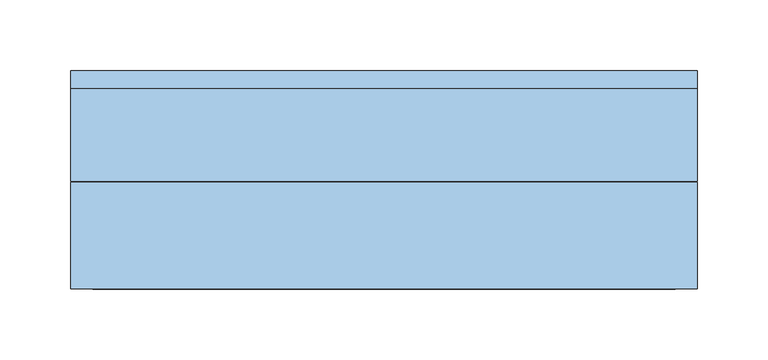
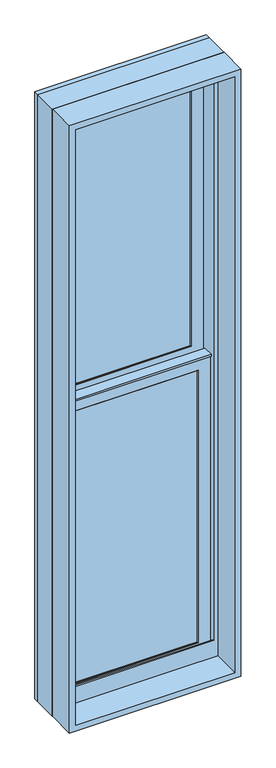
"""IFC4 building model written with IfcOpenShell, lengths in millimetres: window geometry, Window-Double_Hung-Marvin-Essential : ESDH1656."""

from ifc_helpers import new_model, si_unit, frame, origin, place, context, project, spatial, polyline, outline, extrude, faceted_brep, source, transform, mapped, element, save


def window_900ccffd(model_context):
    return source(origin(), model_context, "Body", "SolidModel", [
        extrude(outline(polyline([(64.5583333, 20.6375), (64.5583333, 15.875), (45.5083333, 15.875), (45.5083333, 20.6375), (64.5583333, 20.6375)])), frame((0.0, 0.0, 831.85), z_axis=(0.0, 0.0, 1.0), x_axis=(1.0, 0.0, 0.0)), (0.0, 0.0, 1.0), 755.65),
        extrude(outline(polyline([(-45.5083333, 20.6375), (-45.5083333, 15.875), (-64.5583333, 15.875), (-64.5583333, 20.6375), (-45.5083333, 20.6375)])), frame((0.0, 0.0, 831.85), z_axis=(0.0, 0.0, 1.0), x_axis=(1.0, 0.0, 0.0)), (0.0, 0.0, 1.0), 755.65),
        extrude(outline(polyline([(165.1, 20.6375), (165.1, 15.875), (-165.1, 15.875), (-165.1, 20.6375), (165.1, 20.6375)])), frame((0.0, 0.0, 1200.15), z_axis=(0.0, 0.0, 1.0), x_axis=(1.0, 0.0, 0.0)), (0.0, 0.0, 1.0), 19.05),
        extrude(outline(polyline([(-64.5583333, 46.83125), (-64.5583333, 51.59375), (-45.5083333, 51.59375), (-45.5083333, 46.83125), (-64.5583333, 46.83125)])), frame((0.0, 0.0, 1625.6), z_axis=(0.0, 0.0, 1.0), x_axis=(1.0, 0.0, 0.0)), (0.0, 0.0, 1.0), 755.65),
        extrude(outline(polyline([(45.5083333, 46.83125), (45.5083333, 51.59375), (64.5583333, 51.59375), (64.5583333, 46.83125), (45.5083333, 46.83125)])), frame((0.0, 0.0, 1625.6), z_axis=(0.0, 0.0, 1.0), x_axis=(1.0, 0.0, 0.0)), (0.0, 0.0, 1.0), 755.65),
        extrude(outline(polyline([(-165.1, 46.83125), (-165.1, 51.59375), (165.1, 51.59375), (165.1, 46.83125), (-165.1, 46.83125)])), frame((0.0, 0.0, 1993.9), z_axis=(0.0, 0.0, 1.0), x_axis=(1.0, 0.0, 0.0)), (0.0, 0.0, 1.0), 19.05),
        extrude(outline(polyline([(64.5583333, 20.6375), (45.5083333, 20.6375), (45.5083333, 25.4), (64.5583333, 25.4), (64.5583333, 20.6375)])), frame((0.0, 0.0, 831.85), z_axis=(0.0, 0.0, 1.0), x_axis=(1.0, 0.0, 0.0)), (0.0, 0.0, 1.0), 755.65),
        extrude(outline(polyline([(-45.5083333, 20.6375), (-64.5583333, 20.6375), (-64.5583333, 25.4), (-45.5083333, 25.4), (-45.5083333, 20.6375)])), frame((0.0, 0.0, 831.85), z_axis=(0.0, 0.0, 1.0), x_axis=(1.0, 0.0, 0.0)), (0.0, 0.0, 1.0), 755.65),
        extrude(outline(polyline([(165.1, 20.6375), (-165.1, 20.6375), (-165.1, 25.4), (165.1, 25.4), (165.1, 20.6375)])), frame((0.0, 0.0, 1200.15), z_axis=(0.0, 0.0, 1.0), x_axis=(1.0, 0.0, 0.0)), (0.0, 0.0, 1.0), 19.05),
        extrude(outline(polyline([(-64.5583333, 56.35625), (-45.5083333, 56.35625), (-45.5083333, 51.59375), (-64.5583333, 51.59375), (-64.5583333, 56.35625)])), frame((0.0, 0.0, 1625.6), z_axis=(0.0, 0.0, 1.0), x_axis=(1.0, 0.0, 0.0)), (0.0, 0.0, 1.0), 755.65),
        extrude(outline(polyline([(45.5083333, 56.35625), (64.5583333, 56.35625), (64.5583333, 51.59375), (45.5083333, 51.59375), (45.5083333, 56.35625)])), frame((0.0, 0.0, 1625.6), z_axis=(0.0, 0.0, 1.0), x_axis=(1.0, 0.0, 0.0)), (0.0, 0.0, 1.0), 755.65),
        extrude(outline(polyline([(-165.1, 56.35625), (165.1, 56.35625), (165.1, 51.59375), (-165.1, 51.59375), (-165.1, 56.35625)])), frame((0.0, 0.0, 1993.9), z_axis=(0.0, 0.0, 1.0), x_axis=(1.0, 0.0, 0.0)), (0.0, 0.0, 1.0), 19.05),
        faceted_brep([(-192.0875, 5.6780605, 1617.5351748), (-192.0875, 5.6780605, 1612.9), (192.0875, 5.6780605, 1612.9), (192.0875, 5.6780605, 1617.5351748), (-192.0875, 34.8118605, 1617.5351748), (192.0875, 34.8118605, 1617.5351748), (192.0875, 34.8118605, 1612.9), (-192.0875, 34.8118605, 1612.9), (-192.0875, 30.1625, 1612.9), (-192.0875, 30.1625, 804.8625), (-192.0875, 8.9241104, 804.8625), (-192.0875, 8.9241104, 1612.9), (192.0875, 8.9241104, 1612.9), (192.0875, 30.1625, 1612.9), (192.0875, 8.9241104, 804.8625), (192.0875, 30.1625, 804.8625), (-176.2034752, 11.90625, 1598.6034752), (-176.2034752, 30.1625, 1598.6034752), (176.2034752, 30.1625, 1598.6034752), (176.2034752, 11.90625, 1598.6034752), (-159.54375, 10.4662439, 1581.94375), (-159.54375, 11.90625, 1581.94375), (159.54375, 11.90625, 1581.94375), (159.54375, 10.4662439, 1581.94375), (161.0858834, 8.9241104, 1583.4858834), (-161.0858834, 8.9241104, 1583.4858834), (176.2034752, 30.1625, 820.7465248), (176.2034752, 11.90625, 820.7465248), (159.54375, 11.90625, 837.40625), (159.54375, 10.4662439, 837.40625), (161.0858834, 8.9241104, 835.8641166), (-176.2034752, 30.1625, 820.7465248), (-176.2034752, 11.90625, 820.7465248), (-159.54375, 11.90625, 837.40625), (-159.54375, 10.4662439, 837.40625), (-161.0858834, 8.9241104, 835.8641166)], [[[0, 1, 2, 3]], [[4, 5, 6, 7]], [[1, 0, 4, 7, 8, 9, 10, 11]], [[2, 1, 11, 12]], [[7, 6, 13, 8]], [[3, 2, 12, 14, 15, 13, 6, 5]], [[0, 3, 5, 4]], [[16, 17, 18, 19]], [[20, 21, 22, 23]], [[20, 23, 24, 25]], [[19, 18, 26, 27]], [[23, 22, 28, 29]], [[24, 23, 29, 30]], [[27, 26, 31, 32]], [[29, 28, 33, 34]], [[30, 29, 34, 35]], [[15, 14, 10, 9]], [[15, 9, 8, 13], [18, 17, 31, 26]], [[17, 16, 32, 31]], [[16, 19, 27, 32], [22, 21, 33, 28]], [[21, 20, 34, 33]], [[20, 25, 35, 34]], [[10, 14, 12, 11], [25, 24, 30, 35]]]),
        extrude(outline(polyline([(38.5955581, 1598.6125), (33.5778968, 1598.6125), (33.5778968, 1600.2), (39.9405976, 1600.2), (39.9405976, 1598.6125), (61.515625, 1598.6125), (47.6307501, 1595.2975159), (38.5955581, 1595.2975159), (38.5955581, 1598.6125)])), frame((-192.0875, 0.0, 0.0), z_axis=(1.0, 0.0, 0.0), x_axis=(0.0, 1.0, 0.0)), (0.0, 0.0, 1.0), 384.175),
        faceted_brep([(222.25, 0.0, 774.7), (222.25, 0.0, 2438.4), (-222.25, 0.0, 2438.4), (-222.25, 0.0, 774.7), (196.05625, 0.0, 835.81875), (-196.05625, 0.0, 835.81875), (-196.05625, 0.0, 2412.20625), (196.05625, 0.0, 2412.20625), (196.05625, 3.96875, 774.7), (-196.05625, 3.96875, 774.7), (-196.05625, 3.96875, 835.81875), (196.05625, 3.96875, 835.81875), (-222.25, 65.6828125, 774.7), (-196.05625, 65.6828125, 774.7), (196.05625, 65.6828125, 774.7), (222.25, 65.6828125, 774.7), (-222.25, 65.6828125, 2438.4), (222.25, 65.6828125, 2438.4), (196.05625, 65.6828125, 2412.20625), (-196.05625, 65.6828125, 2412.20625)], [[[0, 1, 2, 3], [4, 5, 6, 7]], [[8, 9, 10, 11]], [[5, 4, 11, 10]], [[0, 3, 12, 13, 9, 8, 14, 15]], [[13, 12, 16, 17, 15, 14, 18, 19]], [[13, 19, 6, 5, 10, 9]], [[7, 6, 19, 18]], [[18, 14, 8, 11, 4, 7]], [[1, 0, 15, 17]], [[2, 1, 17, 16]], [[3, 2, 16, 12]]]),
        faceted_brep([(196.05625, 30.1625, 1606.55), (194.46875, 30.1625, 1606.55), (194.46875, 30.1625, 799.0544613), (196.05625, 30.1625, 799.0544613), (-194.46875, 30.1625, 1606.55), (-196.05625, 30.1625, 1606.55), (-196.05625, 30.1625, 799.0544613), (-194.46875, 30.1625, 799.0544613), (194.46875, 63.5, 1606.55), (196.05625, 63.5, 1606.55), (196.05625, 63.5, 792.5743077), (194.46875, 63.5, 792.5743077), (-196.05625, 63.5, 1606.55), (-194.46875, 63.5, 1606.55), (-194.46875, 63.5, 792.5743077), (-196.05625, 63.5, 792.5743077), (207.3108932, 3.96875, 804.1460105), (207.3108932, 3.96875, 774.7), (207.3108932, 65.6828125, 774.7), (207.3108932, 65.6828125, 792.150012), (-207.3108932, 3.96875, 774.7), (-207.3108932, 3.96875, 804.1460105), (-207.3108932, 65.6828125, 792.150012), (-207.3108932, 65.6828125, 774.7), (207.3108932, 78.58125, 789.6428097), (-207.3108932, 78.58125, 789.6428097), (-205.2971252, 68.2348864, 791.6539391), (-187.33135, 68.2348864, 791.6539391), (-187.33135, 65.6828125, 792.150012), (187.33135, 65.6828125, 792.150012), (187.33135, 68.2348864, 791.6539391), (205.2971252, 68.2348864, 791.6539391), (-222.25, 65.6828125, 774.7), (-222.25, 78.5948249, 774.7), (222.25, 78.5948249, 774.7), (222.25, 65.6828125, 774.7), (-222.25, 78.58125, 2438.4), (222.25, 78.58125, 2438.4), (207.3108932, 78.58125, 2423.4608932), (-207.3108932, 78.58125, 2423.4608932), (-222.25, 65.6828125, 2438.4), (-205.2971252, 68.2348864, 2421.4471252), (205.2971252, 68.2348864, 2421.4471252), (187.33135, 68.2348864, 2403.48135), (-187.33135, 68.2348864, 2403.48135), (-187.33135, 65.6828125, 2403.48135), (187.33135, 65.6828125, 2403.48135), (222.25, 65.6828125, 2438.4)], [[[0, 1, 2, 3]], [[4, 5, 6, 7]], [[8, 9, 10, 11]], [[12, 13, 14, 15]], [[1, 8, 11, 2]], [[9, 0, 3, 10]], [[1, 0, 9, 8]], [[5, 4, 13, 12]], [[5, 12, 15, 6]], [[13, 4, 7, 14]], [[16, 17, 18, 19]], [[20, 21, 22, 23]], [[24, 25, 26, 27, 28, 22, 21, 16, 19, 29, 30, 31], [3, 2, 11, 10], [7, 6, 15, 14]], [[17, 16, 21, 20]], [[17, 20, 23, 32, 33, 34, 35, 18]], [[34, 33, 36, 37], [25, 24, 38, 39]], [[33, 32, 40, 36]], [[39, 41, 26, 25]], [[41, 42, 31, 30, 43, 44, 27, 26]], [[44, 45, 28, 27]], [[40, 32, 23, 22, 28, 45, 46, 29, 19, 18, 35, 47]], [[36, 40, 47, 37]], [[39, 38, 42, 41]], [[44, 43, 46, 45]], [[34, 37, 47, 35]], [[42, 38, 24, 31]], [[46, 43, 30, 29]]]),
        extrude(outline(polyline([(172.24375, 11.90625), (-172.24375, 11.90625), (-172.24375, 15.08125), (172.24375, 15.08125), (172.24375, 11.90625)])), frame((0.0, 0.0, 824.70625), z_axis=(0.0, 0.0, 1.0), x_axis=(1.0, 0.0, 0.0)), (0.0, 0.0, 1.0), 769.9375),
        extrude(outline(polyline([(172.24375, 42.8625), (-172.24375, 42.8625), (-172.24375, 46.0375), (172.24375, 46.0375), (172.24375, 42.8625)])), frame((0.0, 0.0, 1618.45625), z_axis=(0.0, 0.0, 1.0), x_axis=(1.0, 0.0, 0.0)), (0.0, 0.0, 1.0), 769.9375),
        faceted_brep([(-159.54375, 31.194477, 1581.94375), (-161.0858834, 32.7366104, 1583.4858834), (161.0858834, 32.7366104, 1583.4858834), (159.54375, 31.194477, 1581.94375), (-159.54375, 30.1625, 1581.94375), (159.54375, 30.1625, 1581.94375), (-192.0875, 32.7366104, 1614.4875), (-192.0875, 30.1625, 1614.4875), (192.0875, 30.1625, 1614.4875), (192.0875, 32.7366104, 1614.4875), (161.0858834, 32.7366104, 835.8641166), (159.54375, 31.194477, 837.40625), (159.54375, 30.1625, 837.40625), (192.0875, 30.1625, 804.8625), (192.0875, 32.7366104, 804.8625), (-161.0858834, 32.7366104, 835.8641166), (-159.54375, 31.194477, 837.40625), (-159.54375, 30.1625, 837.40625), (-192.0875, 30.1625, 804.8625), (-192.0875, 32.7366104, 804.8625)], [[[0, 1, 2, 3]], [[4, 0, 3, 5]], [[6, 7, 8, 9]], [[3, 2, 10, 11]], [[5, 3, 11, 12]], [[9, 8, 13, 14]], [[11, 10, 15, 16]], [[12, 11, 16, 17]], [[14, 13, 18, 19]], [[9, 14, 19, 6], [1, 15, 10, 2]], [[16, 15, 1, 0]], [[17, 16, 0, 4]], [[7, 18, 13, 8], [5, 12, 17, 4]], [[19, 18, 7, 6]]]),
        faceted_brep([(-176.2034752, 42.8625, 2392.3534752), (-176.2034752, 61.11875, 2392.3534752), (176.2034752, 61.11875, 2392.3534752), (176.2034752, 42.8625, 2392.3534752), (-159.54375, 41.4224939, 2375.69375), (-159.54375, 42.8625, 2375.69375), (159.54375, 42.8625, 2375.69375), (159.54375, 41.4224939, 2375.69375), (-161.0858834, 39.8803604, 2377.2358834), (161.0858834, 39.8803604, 2377.2358834), (-192.0875, 61.11875, 2408.2375), (-192.0875, 39.8803604, 2408.2375), (192.0875, 39.8803604, 2408.2375), (192.0875, 61.11875, 2408.2375), (176.2034752, 61.11875, 1614.4965248), (176.2034752, 42.8625, 1614.4965248), (159.54375, 42.8625, 1631.15625), (159.54375, 41.4224939, 1631.15625), (161.0858834, 39.8803604, 1629.6141166), (192.0875, 39.8803604, 1598.6125), (192.0875, 61.11875, 1598.6125), (-176.2034752, 61.11875, 1614.4965248), (-176.2034752, 42.8625, 1614.4965248), (-159.54375, 42.8625, 1631.15625), (-159.54375, 41.4224939, 1631.15625), (-161.0858834, 39.8803604, 1629.6141166), (-192.0875, 39.8803604, 1598.6125), (-192.0875, 61.11875, 1598.6125)], [[[0, 1, 2, 3]], [[4, 5, 6, 7]], [[8, 4, 7, 9]], [[10, 11, 12, 13]], [[3, 2, 14, 15]], [[7, 6, 16, 17]], [[9, 7, 17, 18]], [[13, 12, 19, 20]], [[15, 14, 21, 22]], [[17, 16, 23, 24]], [[18, 17, 24, 25]], [[20, 19, 26, 27]], [[13, 20, 27, 10], [1, 21, 14, 2]], [[22, 21, 1, 0]], [[3, 15, 22, 0], [5, 23, 16, 6]], [[24, 23, 5, 4]], [[25, 24, 4, 8]], [[11, 26, 19, 12], [9, 18, 25, 8]], [[27, 26, 11, 10]]]),
        faceted_brep([(-192.0875, 61.11875, 1598.6125), (-192.0875, 63.6928604, 1598.6125), (192.0875, 63.6928604, 1598.6125), (192.0875, 61.11875, 1598.6125), (-159.54375, 62.150727, 1631.15625), (-159.54375, 61.11875, 1631.15625), (159.54375, 61.11875, 1631.15625), (159.54375, 62.150727, 1631.15625), (-161.0858834, 63.6928604, 1629.6141166), (161.0858834, 63.6928604, 1629.6141166), (192.0875, 63.6928604, 2408.2375), (192.0875, 61.11875, 2408.2375), (159.54375, 61.11875, 2375.69375), (159.54375, 62.150727, 2375.69375), (161.0858834, 63.6928604, 2377.2358834), (-192.0875, 63.6928604, 2408.2375), (-192.0875, 61.11875, 2408.2375), (-159.54375, 61.11875, 2375.69375), (-159.54375, 62.150727, 2375.69375), (-161.0858834, 63.6928604, 2377.2358834)], [[[0, 1, 2, 3]], [[4, 5, 6, 7]], [[8, 4, 7, 9]], [[3, 2, 10, 11]], [[7, 6, 12, 13]], [[9, 7, 13, 14]], [[11, 10, 15, 16]], [[13, 12, 17, 18]], [[14, 13, 18, 19]], [[16, 15, 1, 0]], [[3, 11, 16, 0], [5, 17, 12, 6]], [[18, 17, 5, 4]], [[19, 18, 4, 8]], [[1, 15, 10, 2], [9, 14, 19, 8]]]),
        extrude(outline(polyline([(172.24375, 26.19375), (-172.24375, 26.19375), (-172.24375, 30.1625), (172.24375, 30.1625), (172.24375, 26.19375)])), frame((0.0, 0.0, 824.70625), z_axis=(0.0, 0.0, 1.0), x_axis=(1.0, 0.0, 0.0)), (0.0, 0.0, 1.0), 769.9375),
        extrude(outline(polyline([(172.24375, 57.15), (-172.24375, 57.15), (-172.24375, 61.11875), (172.24375, 61.11875), (172.24375, 57.15)])), frame((0.0, 0.0, 1618.45625), z_axis=(0.0, 0.0, 1.0), x_axis=(1.0, 0.0, 0.0)), (0.0, 0.0, 1.0), 769.9375),
        extrude(outline(polyline([(2438.4, 222.25), (2438.4, -222.25), (774.7, -222.25), (774.7, 222.25), (2438.4, 222.25)]), holes=[polyline([(2422.525, 206.375), (790.575, 206.375), (790.575, -206.375), (2422.525, -206.375), (2422.525, 206.375)])]), frame((0.0, -76.2, 0.0), z_axis=(0.0, 1.0, 0.0), x_axis=(0.0, 0.0, 1.0)), (0.0, 0.0, 1.0), 75.40625),
    ])


if __name__ == "__main__":
    model = new_model("IFC4")
    model_context = context("Model", 3, world=origin())
    ifc_project = project(units=[si_unit("LENGTHUNIT", "METRE", prefix="MILLI")], contexts=[model_context])
    site = spatial("IfcSite", under=ifc_project)
    building = spatial("IfcBuilding", under=site)
    placement = place(None, origin())
    window_shape = window_900ccffd(model_context)
    element("IfcWindow", 1, ObjectType="Window-Double_Hung-Marvin-Essential : ESDH1656", at=placement, inside=building, context=model_context, shape_type="MappedRepresentation", body=[
        mapped(window_shape, transform((0.0, 0.0, 0.0), x_axis=(1.0, 0.0, 0.0), y_axis=(0.0, 1.0, 0.0), z_axis=(0.0, 0.0, 1.0))),
    ])
    save(model, "model.ifc")

# Revit data of these elements
# Type "Window-Double_Hung-Marvin-Essential : ESDH1656"
#   Type Mark = "68"
#   Window Type = "Essential Double Hung"
#   Product data url = "https://bimobject.com/marvin-windows-and-doors/product/marvin-dhwau"
#   Product Guid = "c4a96547-874c-4385-91dc-a058adc19d98"
#   Frame = "All Ultrex"
#   Egress Window = "No"
#   URL = "www.marvin.com"
#   Model = "ESDH1656"
#   Manufacturer = "Marvin Windows and Doors"
#   Label Egress = ""
#   Glass Type = "IG Low E II with Argon"
#   Design Pressure = "DP40"
#   Description = "1866 DBHG"
#   Analytic Construction = "<None>"
#   Prairie Corner Width = 0' - 4"
#   Prairie Corner Height = 0' - 4"
#   Egress Width = 1' - 2 9/16"
#   Egress Height = 2' - 4 27/128"
#   Rough Width = 1' - 6"
#   Rough Height = 5' - 6"
#   Nominal Width = 1' - 6"
#   Nominal Height = 5' - 6"
#   Inset to Installation Flange [instance default] = 0' - 1"
#   Height = 5' - 5 1/2"
#   Egress Area = 2.85293 SF
#   Default Head Height = 8' - 0"
#   Width = 1' - 5 1/2"
#   Daylight Area = 5.11442 SF
#   DLO Width = 1' - 0 9/16"
#   DLO Height = 2' - 5 5/16"
#   Muntins Top Sash = yes
#   Lites Wide Top Sash = 3
#   Lites Wide Bottom Sash = 3
#   Lites High Top Sash = 2
#   Lites High Bottom Sash = 2
#   Lite Cut Prairie 9 = no
#   Lite Cut HV Grid = yes
#   Muntins Bottom Sash = yes
#   Label Visibility = no
#   Jamb Extension Visibility = yes
#   Edition number = 1
#   Interior Material = Ultrex-Marvin-Stonewhite
#   Glazing Material = Glass-Marvin-IG Low E II with Argon
#   Cladding Material = Ultrex-Marvin-Pebblegray
#   Wall Closure = (empty or 0)
#   Assembly Code = ""
# Element 1 (IfcWindow, "Window-Double_Hung-Marvin-Essential : ESDH1656")
#   Materials on its faces: "Ultrex-Marvin-Pebblegray", "Ultrex-Marvin-Stonewhite", "Glass-Marvin-IG Low E II with Argon"
# Materials
#   "Ultrex-Marvin-Stonewhite": class "Paint", colour RGB 250 251 245, transparency 0
#   "Glass-Marvin-IG Low E II with Argon": class "Glass", colour RGB 0 128 192, transparency 0.85
#   "Ultrex-Marvin-Pebblegray": class "Paint", colour RGB 189 185 173, transparency 0
